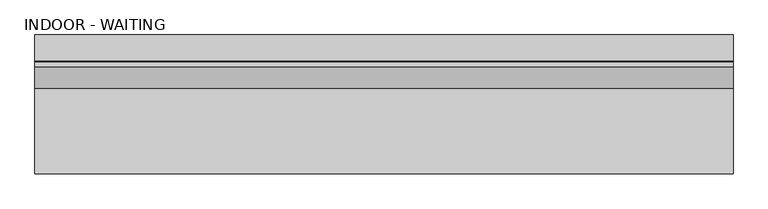
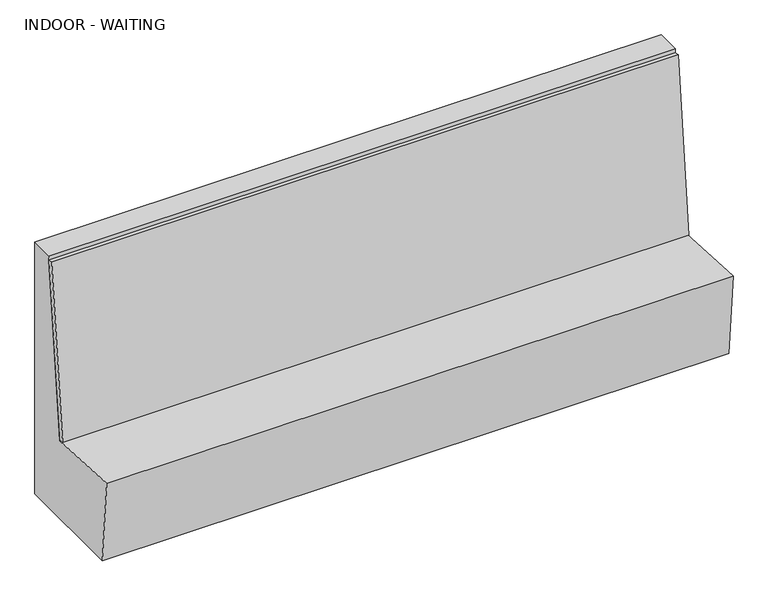
"""IFC4 building model written with IfcOpenShell, lengths in millimetres: furniture geometry, OD_CW_Booth : INDOOR - WAITING."""

from ifc_helpers import new_model, si_unit, frame, origin, place, context, project, spatial, polyline, outline, extrude, source, transform, mapped, element, save


def indoor_waiting_798d4b4b(model_context):
    return source(origin(), model_context, "Body", "SweptSolid", [
        extrude(outline(polyline([(0.0, 3286.7570278), (25.4, 3286.7570278), (25.4, 0.0), (0.0, 0.0), (0.0, 3286.7570278)])), frame((3305.4947327, 358.2049359, 438.8309433), z_axis=(0.0, 0.10452846326765197, 0.9945218953682735), x_axis=(0.0, 0.9945218953682735, -0.10452846326765197)), (0.0, 0.0, 1.0), 944.7333479),
        extrude(outline(polyline([(609.6, 1397.0), (609.6, 0.0), (-3.4100193, 0.0), (-43.0849153, 453.4861359), (382.9385128, 431.1591941), (484.4524721, 1397.0), (609.6, 1397.0)])), frame((18.7377049, 0.0, 0.0), z_axis=(1.0, 0.0, 0.0), x_axis=(0.0, 1.0, 0.0)), (0.0, 0.0, 1.0), 3286.7570278),
    ])


if __name__ == "__main__":
    model = new_model("IFC4")
    model_context = context("Model", 3, world=origin())
    ifc_project = project(units=[si_unit("LENGTHUNIT", "METRE", prefix="MILLI")], contexts=[model_context])
    site = spatial("IfcSite", under=ifc_project)
    building = spatial("IfcBuilding", under=site)
    placement = place(None, origin())
    indoor_waiting_shape = indoor_waiting_798d4b4b(model_context)
    element("IfcFurniture", 1, ObjectType="OD_CW_Booth : INDOOR - WAITING", at=placement, inside=building, context=model_context, shape_type="MappedRepresentation", body=[
        mapped(indoor_waiting_shape, transform((0.0, 0.0, 0.0), x_axis=(1.0, 0.0, 0.0), y_axis=(0.0, 1.0, 0.0), z_axis=(0.0, 0.0, 1.0))),
    ])
    save(model, "model.ifc")

# Revit data of these elements
# Type "OD_CW_Booth : INDOOR - WAITING"
#   Width = 4' - 0"
#   OD_CW_Width [instance default] = 2' - 10"
#   OD_CW_Length [instance default] = 26' - 1 83/256"
#   OD_CW_Height [instance default] = 2' - 3"
#   Height = 3' - 0"
#   Depth = 2' - 0"
#   Seating Count [instance default] = 10
#   back = WOOD VENEER
#   OD_CW_Material_Front Panel [instance default] = none
#   OD_CW_Material_Body [instance default] = none
# Element 1 (IfcFurniture, "OD_CW_Booth : INDOOR - WAITING")
#   OD_CW_Length = 10' - 9.39988"
#   Seating Count = 4
#   OD_CW_Material_Body = WOOD-OAKFIRE
#   Materials on its faces: "WOOD-OAKFIRE", "WOOD VENEER"
# Materials
#   "WOOD VENEER": class "Miscellaneous", colour RGB 164 164 164, transparency 0, Cost = 0
#   "WOOD-OAKFIRE": class "Wood", colour RGB 198 202 183, transparency 0, Description = "Generic wood", Cost = 0
